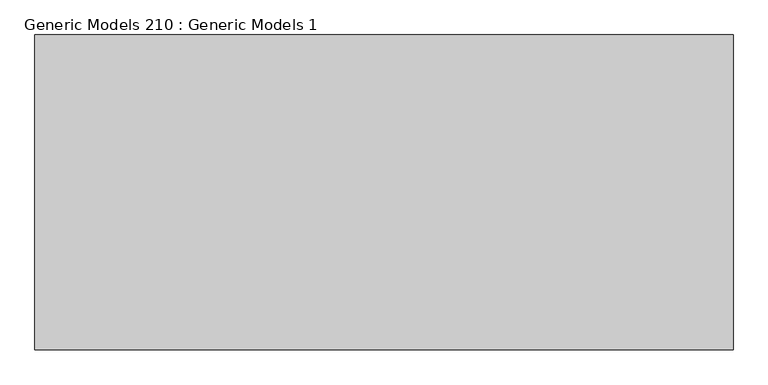
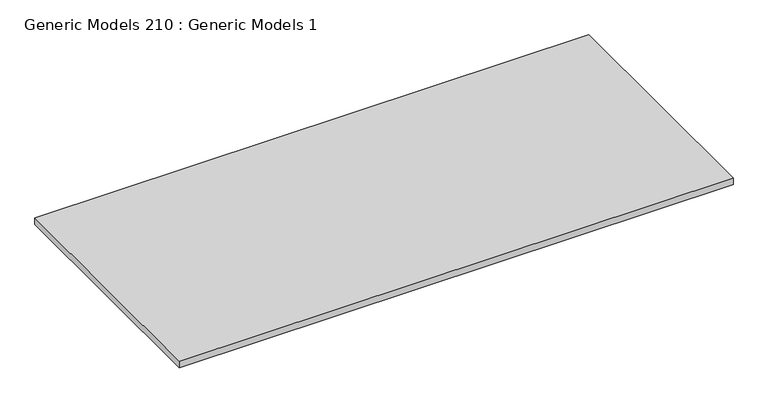
"""IFC4 building model written with IfcOpenShell, lengths in millimetres: proxy geometry, Generic Models 210 : Generic Models 1."""

from ifc_helpers import new_model, si_unit, frame, origin, place, context, project, spatial, polyline, outline, extrude, source, transform, mapped, element, save


def generic_models_210_generic_models_1_57077528(model_context):
    return source(origin(), model_context, "Body", "SweptSolid", [
        extrude(outline(polyline([(-1609.6874339, 1085.2769662), (-89.0736296, 1085.2769662), (-89.0736296, 399.7309662), (-1609.6874339, 399.7309662), (-1609.6874339, 1085.2769662)])), frame((0.0, 0.0, 126783.846), z_axis=(0.0, 0.0, 1.0), x_axis=(1.0, 0.0, 0.0)), (0.0, 0.0, 1.0), 19.05),
    ])


if __name__ == "__main__":
    model = new_model("IFC4")
    model_context = context("Model", 3, world=origin())
    ifc_project = project(units=[si_unit("LENGTHUNIT", "METRE", prefix="MILLI")], contexts=[model_context])
    site = spatial("IfcSite", under=ifc_project)
    building = spatial("IfcBuilding", under=site)
    placement = place(None, origin())
    generic_models_210_generic_models_1_shape = generic_models_210_generic_models_1_57077528(model_context)
    element("IfcBuildingElementProxy", 1, Name="Generic Models 210 : Generic Models 1", ObjectType="Generic Models 210 : Generic Models 1", at=placement, inside=building, context=model_context, shape_type="MappedRepresentation", body=[
        mapped(generic_models_210_generic_models_1_shape, transform((0.0, 0.0, 0.0), x_axis=(1.0, 0.0, 0.0), y_axis=(0.0, 1.0, 0.0), z_axis=(0.0, 0.0, 1.0))),
    ])
    save(model, "model.ifc")

# Revit data of these elements
# Element 1 (IfcBuildingElementProxy, "Generic Models 210 : Generic Models 1")
#   Materials on its faces: "_WOOD FLOORING (SPEC T.B.D.)"
# Materials
#   "_WOOD FLOORING (SPEC T.B.D.)": class "Generic", colour RGB 177 130 114, transparency 0, Cost = 0
